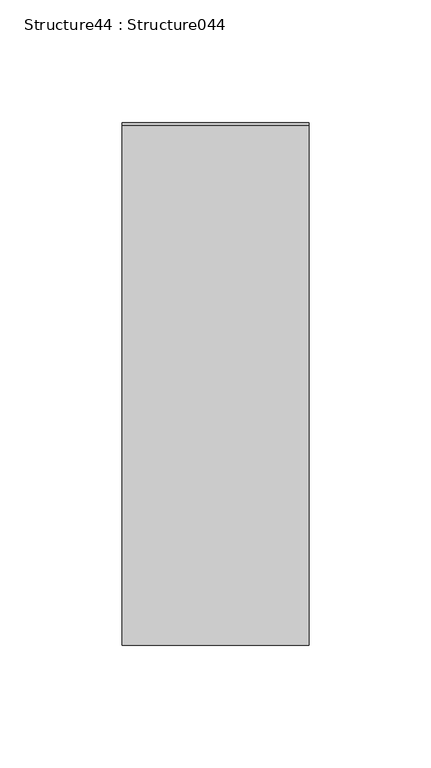
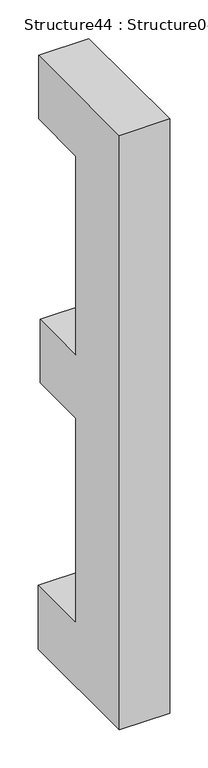
"""IFC4 building model written with IfcOpenShell, lengths in millimetres: proxy geometry, Structure44 : Structure044."""

from ifc_helpers import new_model, si_unit, frame, origin, place, context, project, spatial, polyline, outline, extrude, source, transform, mapped, element, save


def structure44_structure044_871b3205(model_context):
    return source(origin(), model_context, "Body", "SweptSolid", [
        extrude(outline(polyline([(251506.8455788, 4480.4419946), (251718.9780705, 4480.4419946), (251718.9780705, 4378.4602217), (251621.0817153, 4378.4602217), (251621.0817153, 4060.2611693), (251714.8932827, 4060.2611693), (251714.8932827, 3958.2800261), (251621.0817153, 3958.2800261), (251621.0817153, 3630.5630275), (251720.3339984, 3630.5630275), (251720.3339984, 3528.5825142), (251506.8455788, 3528.5825142), (251506.8455788, 4480.4419946)])), frame((-38594.2176606, 0.0, 0.0), z_axis=(1.0, 0.0, 0.0), x_axis=(0.0, 1.0, 0.0)), (0.0, 0.0, 1.0), 76.2),
    ])


if __name__ == "__main__":
    model = new_model("IFC4")
    model_context = context("Model", 3, world=origin())
    ifc_project = project(units=[si_unit("LENGTHUNIT", "METRE", prefix="MILLI")], contexts=[model_context])
    site = spatial("IfcSite", under=ifc_project)
    building = spatial("IfcBuilding", under=site)
    placement = place(None, origin())
    structure44_structure044_shape = structure44_structure044_871b3205(model_context)
    element("IfcBuildingElementProxy", 1, Name="Structure44 : Structure044", ObjectType="Structure44 : Structure044", at=placement, inside=building, context=model_context, shape_type="MappedRepresentation", body=[
        mapped(structure44_structure044_shape, transform((0.0, 0.0, 0.0), x_axis=(1.0, 0.0, 0.0), y_axis=(0.0, 1.0, 0.0), z_axis=(0.0, 0.0, 1.0))),
    ])
    save(model, "model.ifc")

# Revit data of these elements
# Type "Structure44 : Structure044"
#   NameOverride = "Structure044"
# Element 1 (IfcBuildingElementProxy, "Structure44 : Structure044")
#   Materials on its faces: "BRUSHED ALUM. LETTERING"
# Materials
#   "BRUSHED ALUM. LETTERING": class "Unassigned", colour RGB 169 181 186, transparency 0, Cost = 0
